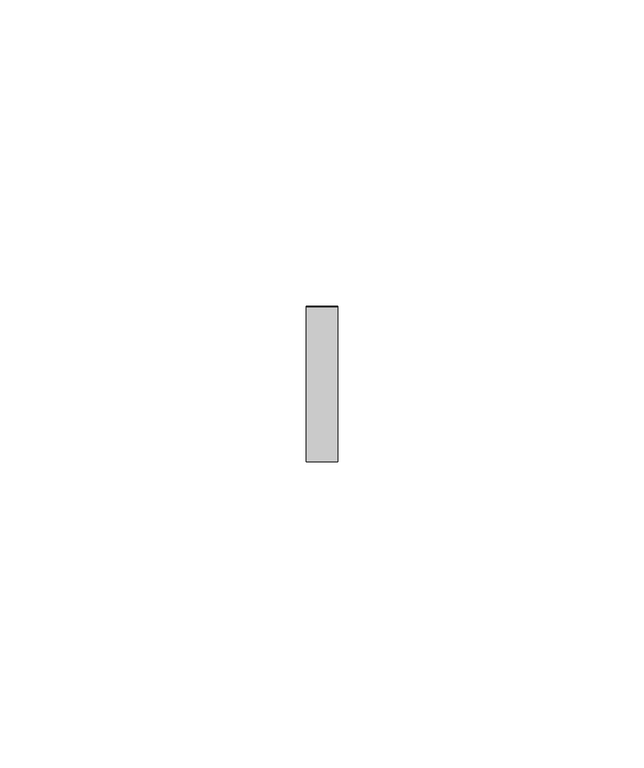
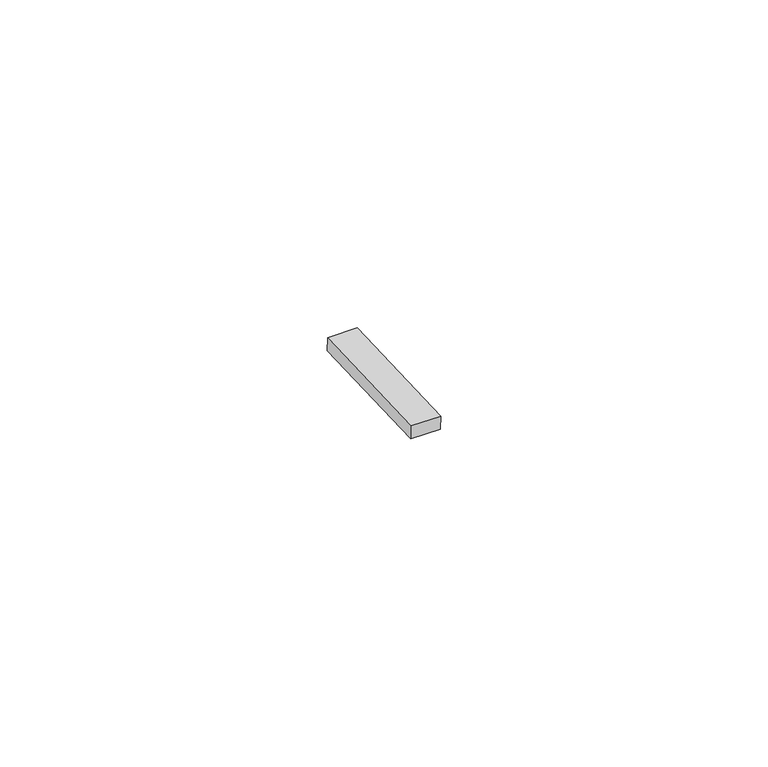
"""IFC4 building model written with IfcOpenShell, lengths in millimetres: proxy geometry, Inner panel:Inner panel:1:Inner panel:1 : Inner panel:Inner panel:300324:2:Inner panel:1:Inner panel:1 : Inner panel:Inner panel:300324:2 : Inner panel:Inner panel:1:Inner panel:1 : Inner panel:Inner panel:300324:300043:120 : Inner panel:Inner panel:1:Inner panel:1 : Inner panel:Inner panel:300324:2:Inner panel:1:Inner panel:1 : Inner panel:Inner panel:300324:2 : Inner panel:Inner panel:1:Inner panel:1 : Inner panel:Inner panel:300324:300043:308120."""

from ifc_helpers import new_model, si_unit, frame, origin, place, context, project, spatial, polyline, outline, extrude, source, transform, mapped, element, save


def generic_models_16201368(model_context):
    return source(origin(), model_context, "Body", "SweptSolid", [
        extrude(outline(polyline([(0.0, -25.3999999), (0.0, 0.0), (5.2138089, 0.0), (5.2138089, -25.3999999), (0.0, -25.3999999)])), frame((592310.995117, -578962.7476805, 3951.4793391), z_axis=(0.0, -0.041630544712223896, 0.9991330730923502), x_axis=(-1.0, 0.0, 0.0)), (0.0, 0.0, 1.0), 2.4763745),
    ])


if __name__ == "__main__":
    model = new_model("IFC4")
    model_context = context("Model", 3, world=origin())
    ifc_project = project(units=[si_unit("LENGTHUNIT", "METRE", prefix="MILLI")], contexts=[model_context])
    site = spatial("IfcSite", under=ifc_project)
    building = spatial("IfcBuilding", under=site)
    placement = place(None, origin())
    generic_models_shape = generic_models_16201368(model_context)
    element("IfcBuildingElementProxy", 1, Name="Inner panel:Inner panel:1:Inner panel:1 : Inner panel:Inner panel:300324:2:Inner panel:1:Inner panel:1 : Inner panel:Inner panel:300324:2 : Inner panel:Inner panel:1:Inner panel:1 : Inner panel:Inner panel:300324:300043:120 : Inner panel:Inner panel:1:Inner panel:1 : Inner panel:Inner panel:300324:2:Inner panel:1:Inner panel:1 : Inner panel:Inner panel:300324:2 : Inner panel:Inner panel:1:Inner panel:1 : Inner panel:Inner panel:300324:300043:308120", ObjectType="Inner panel:Inner panel:1:Inner panel:1 : Inner panel:Inner panel:300324:2:Inner panel:1:Inner panel:1 : Inner panel:Inner panel:300324:2 : Inner panel:Inner panel:1:Inner panel:1 : Inner panel:Inner panel:300324:300043:120 : Inner panel:Inner panel:1:Inner panel:1 : Inner panel:Inner panel:300324:2:Inner panel:1:Inner panel:1 : Inner panel:Inner panel:300324:2 : Inner panel:Inner panel:1:Inner panel:1 : Inner panel:Inner panel:300324:300043:308120", at=placement, inside=building, context=model_context, shape_type="MappedRepresentation", body=[
        mapped(generic_models_shape, transform((0.0, 0.0, 0.0), x_axis=(1.0, 0.0, 0.0), y_axis=(0.0, 1.0, 0.0), z_axis=(0.0, 0.0, 1.0))),
    ])
    save(model, "model.ifc")

# Revit data of these elements
# Type "Inner panel:Inner panel:1:Inner panel:1 : Inner panel:Inner panel:300324:2:Inner panel:1:Inner panel:1 : Inner panel:Inner panel:300324:2 : Inner panel:Inner panel:1:Inner panel:1 : Inner panel:Inner panel:300324:300043:120 : Inner panel:Inner panel:1:Inner panel:1 : Inner panel:Inner panel:300324:2:Inner panel:1:Inner panel:1 : Inner panel:Inner panel:300324:2 : Inner panel:Inner panel:1:Inner panel:1 : Inner panel:Inner panel:300324:300043:308120"
#   NameOverride = "Inner panel:Inner panel:1:Inner panel:1 : Inner panel:Inner panel:300324:2:Inner panel:1:Inner panel:1 : Inner panel:Inner panel:300324:2 : Inner panel:Inner panel:1:Inner panel:1 : Inner panel:Inner panel:300324:300043:308120"
#   ObjectTypeOverride = "Inner panel:1:Inner panel:1 : Inner panel:Inner panel:300324:2 : Inner panel:Inner panel:1:Inner panel:1 : Inner panel:Inner panel:300324:300043"
#   Reference = "Inner panel"
#   Tag = "308120"
# Element 1 (IfcBuildingElementProxy, "Inner panel:Inner panel:1:Inner panel:1 : Inner panel:Inner panel:300324:2:Inner panel:1:Inner panel:1 : Inner panel:Inner panel:300324:2 : Inner panel:Inner panel:1:Inner panel:1 : Inner panel:Inner panel:300324:300043:120 : Inner panel:Inner panel:1:Inner panel:1 : Inner panel:Inner panel:300324:2:Inner panel:1:Inner panel:1 : Inner panel:Inner panel:300324:2 : Inner panel:Inner panel:1:Inner panel:1 : Inner panel:Inner panel:300324:300043:308120")
#   Materials on its faces: "AT CLIP - 1\" WIDE NON ABSORBENT, WEATHER-RESISTANT NEOPRENE/EPDM/SBR FOAM"
# Materials
#   "AT CLIP - 1\" WIDE NON ABSORBENT, WEATHER-RESISTANT NEOPRENE/EPDM/SBR FOAM": class "Generic", colour RGB 85 85 85, transparency 0, Cost = 0
